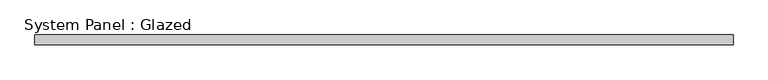
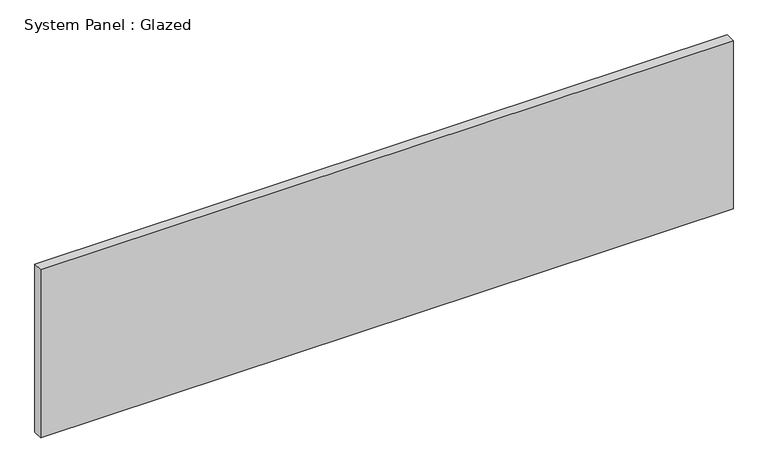
"""IFC4 building model written with IfcOpenShell, lengths in millimetres: plate geometry, System Panel : Glazed."""

from ifc_helpers import new_model, si_unit, origin, origin_with_axes, place, context, project, spatial, polyline, outline, extrude, source, transform, mapped, element, save


def system_panel_glazed_bd903948(model_context):
    return source(origin(), model_context, "Body", "SweptSolid", [
        extrude(outline(polyline([(877.5, -49.5), (-877.5, -49.5), (-877.5, -24.5), (877.5, -24.5), (877.5, -49.5)])), origin_with_axes(), (0.0, 0.0, 1.0), 450.0),
    ])


if __name__ == "__main__":
    model = new_model("IFC4")
    model_context = context("Model", 3, world=origin())
    ifc_project = project(units=[si_unit("LENGTHUNIT", "METRE", prefix="MILLI")], contexts=[model_context])
    site = spatial("IfcSite", under=ifc_project)
    building = spatial("IfcBuilding", under=site)
    placement = place(None, origin())
    system_panel_glazed_shape = system_panel_glazed_bd903948(model_context)
    element("IfcPlate", 1, ObjectType="System Panel : Glazed", at=placement, inside=building, context=model_context, shape_type="MappedRepresentation", body=[
        mapped(system_panel_glazed_shape, transform((0.0, 0.0, 0.0), x_axis=(1.0, 0.0, 0.0), y_axis=(0.0, 1.0, 0.0), z_axis=(0.0, 0.0, 1.0))),
    ])
    save(model, "model.ifc")

# Revit data of these elements
# Type "System Panel : Glazed"
#   Keynote = "H11"
#   Construction Type Id = "GSP4R"
#   Analytic Construction = "1/8 in Pilkington single glazing"
#   Visual Light Transmittance = 0.9
#   Solar Heat Gain Coefficient = 0.86
#   Heat Transfer Coefficient (U) = 6.7069 W/(m²·K)
# Element 1 (IfcPlate, "System Panel : Glazed")
#   Materials on its faces: "Glass"
# Materials
#   "Glass": class "Glass", colour RGB 0 128 192, transparency 0.9, Description = "Soda Lime Glass", Cost = 0
